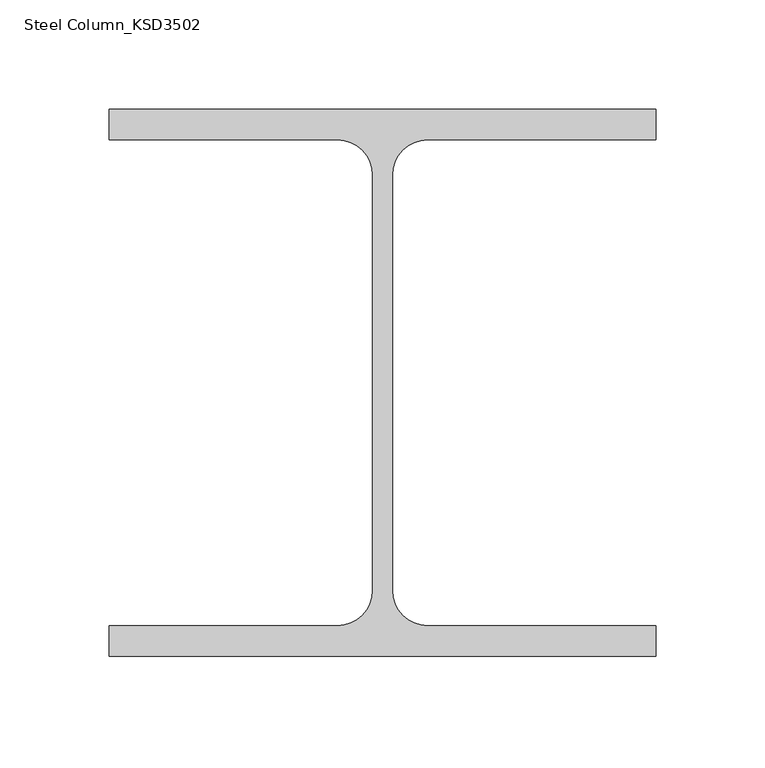
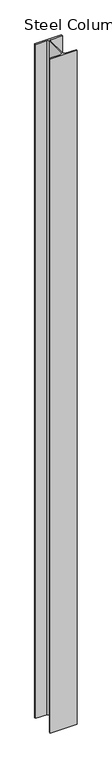
"""IFC4 building model written with IfcOpenShell, lengths in millimetres: column geometry, Steel Column_KSD3502 : H_SC_ASC_H-250×250x9x14."""

import ifcopenshell
import ifcopenshell.guid

model = None  # the IFC model being written
_history = None  # IfcOwnerHistory: only IFC2X3 demands one
_inside = {}  # id of a spatial element -> (the spatial element, [elements in it])
_under = {}  # id of a project, library or spatial element -> (it, [spatial elements below it])
_declared = {}  # id of a project -> (the project, [libraries it declares])
_typed = {}  # id of a type object -> (the type object, [elements of that type])
_made_of = {}  # id of a material, layer set ... -> (it, [elements and type objects made of it])


def new_model(schema):
    """Start an empty IFC model of exactly this schema.

    Asked for "IFC4X3", IfcOpenShell would pick the latest addendum, in which some entities
    have other attributes; the version numbers below select the first issue.
    IFC2X3 requires an IfcOwnerHistory on every rooted entity: one is made here for all.
    """
    global model, _history
    if schema == "IFC4X3":
        model = ifcopenshell.file(schema_version=(4, 3, 0, 0))
    else:
        model = ifcopenshell.file(schema=schema)
    _inside.clear()
    _under.clear()
    _declared.clear()
    _typed.clear()
    _made_of.clear()
    _history = None
    if model.schema == "IFC2X3":
        org = make("IfcOrganization", Name="unknown")
        user = make(
            "IfcPersonAndOrganization",
            ThePerson=make("IfcPerson", FamilyName="unknown"),
            TheOrganization=org,
        )
        app = make(
            "IfcApplication",
            ApplicationDeveloper=org,
            Version="unknown",
            ApplicationFullName="unknown",
            ApplicationIdentifier="unknown",
        )
        _history = make(
            "IfcOwnerHistory",
            OwningUser=user,
            OwningApplication=app,
            ChangeAction="ADDED",
            CreationDate=0,
        )
    return model


def make(cls, **values):
    """One entity of the class cls with the attributes given. An attribute that is None is left unset."""
    return model.create_entity(
        cls, **{name: value for name, value in values.items() if value is not None}
    )


def rooted(cls, **values):
    """An entity with a GlobalId (a new one), such as an element, a storey or a relation."""
    return make(cls, GlobalId=ifcopenshell.guid.new(), OwnerHistory=_history, **values)


def si_unit(unit_type, name, prefix=None):
    """IfcSIUnit, for example si_unit("LENGTHUNIT", "METRE", prefix="MILLI")."""
    return make("IfcSIUnit", UnitType=unit_type, Prefix=prefix, Name=name)


def assignment(units):
    """IfcUnitAssignment: the units of a project."""
    return None if units is None else make("IfcUnitAssignment", Units=units)


def point(xyz):
    """IfcCartesianPoint."""
    return None if xyz is None else make("IfcCartesianPoint", Coordinates=xyz)


def direction(xyz):
    """IfcDirection."""
    return None if xyz is None else make("IfcDirection", DirectionRatios=xyz)


def frame(location, z_axis=None, x_axis=None):
    """IfcAxis2Placement3D, a coordinate frame: its origin and axes. An axis left out is left unset."""
    return make(
        "IfcAxis2Placement3D",
        Location=point(location),
        Axis=direction(z_axis),
        RefDirection=direction(x_axis),
    )


def frame_2d(location, x_axis=None):
    """IfcAxis2Placement2D, a coordinate frame in the plane: its origin and x axis."""
    return make(
        "IfcAxis2Placement2D", Location=point(location), RefDirection=direction(x_axis)
    )


def origin():
    """The frame at (0, 0, 0) with its axes left unset."""
    return frame((0.0, 0.0, 0.0))


def place(relative_to, where):
    """IfcLocalPlacement: puts the frame where relative to a parent placement (None: the world)."""
    return make(
        "IfcLocalPlacement", PlacementRelTo=relative_to, RelativePlacement=where
    )


def context(
    kind, dimensions, precision=None, world=None, true_north=None, identifier=None
):
    """IfcGeometricRepresentationContext, for example the 3D "Model" context."""
    return make(
        "IfcGeometricRepresentationContext",
        ContextIdentifier=identifier,
        ContextType=kind,
        CoordinateSpaceDimension=dimensions,
        Precision=precision,
        WorldCoordinateSystem=world,
        TrueNorth=true_north,
    )


def project(units=None, contexts=None):
    """IfcProject with its units and contexts."""
    return rooted(
        "IfcProject",
        Name="project",
        RepresentationContexts=contexts,
        UnitsInContext=assignment(units),
    )


def spatial(cls, under=None, at=None, **own):
    """A site, building, storey or space (cls), placed at a placement, below another one or the project."""
    s = rooted(cls, ObjectPlacement=at, **own)
    if under is not None:
        _under.setdefault(under.id(), (under, []))[1].append(s)
    return s


def polyline(points):
    """IfcPolyline through the points."""
    return make("IfcPolyline", Points=[point(p) for p in points])


def circle_curve(where, radius):
    """IfcCircle in the frame where."""
    return make("IfcCircle", Position=where, Radius=radius)


def trimmed(basis, trim1, trim2, sense, master):
    """IfcTrimmedCurve: the piece of a basis curve between two trims."""
    return make(
        "IfcTrimmedCurve",
        BasisCurve=basis,
        Trim1=trim1,
        Trim2=trim2,
        SenseAgreement=sense,
        MasterRepresentation=master,
    )


def segment(curve, same_sense, transition):
    """IfcCompositeCurveSegment."""
    return make(
        "IfcCompositeCurveSegment",
        Transition=transition,
        SameSense=same_sense,
        ParentCurve=curve,
    )


def composite_curve(segments, self_intersect=None):
    """IfcCompositeCurve: segments joined end to end."""
    return make("IfcCompositeCurve", Segments=segments, SelfIntersect=self_intersect)


def outline(outer, holes=None, kind="AREA"):
    """IfcArbitraryClosedProfileDef: a profile drawn as a closed curve; with holes, ...WithVoids."""
    if holes is None:
        return make("IfcArbitraryClosedProfileDef", ProfileType=kind, OuterCurve=outer)
    return make(
        "IfcArbitraryProfileDefWithVoids",
        ProfileType=kind,
        OuterCurve=outer,
        InnerCurves=holes,
    )


def extrude(swept, where, along, depth):
    """IfcExtrudedAreaSolid: the profile swept, set in the frame where, extruded along a direction by depth."""
    return make(
        "IfcExtrudedAreaSolid",
        SweptArea=swept,
        Position=where,
        ExtrudedDirection=direction(along),
        Depth=depth,
    )


def shape(context_of_items, identifier, shape_type, items):
    """IfcShapeRepresentation: the items that make up one representation, for example the "Body"."""
    return make(
        "IfcShapeRepresentation",
        ContextOfItems=context_of_items,
        RepresentationIdentifier=identifier,
        RepresentationType=shape_type,
        Items=items,
    )


def source(mapping_origin, context_of_items, identifier, shape_type, items):
    """IfcRepresentationMap: a shape defined once, which mapped items show again and again."""
    return make(
        "IfcRepresentationMap",
        MappingOrigin=mapping_origin,
        MappedRepresentation=shape(context_of_items, identifier, shape_type, items),
    )


def transform(
    local_origin,
    x_axis=None,
    y_axis=None,
    z_axis=None,
    scale=None,
    scale2=None,
    scale3=None,
    uniform=True,
):
    """IfcCartesianTransformationOperator3D, or its non-uniform kind. x_axis, y_axis, z_axis: its Axis1, 2, 3."""
    if uniform:
        return make(
            "IfcCartesianTransformationOperator3D",
            Axis1=direction(x_axis),
            Axis2=direction(y_axis),
            LocalOrigin=point(local_origin),
            Scale=scale,
            Axis3=direction(z_axis),
        )
    return make(
        "IfcCartesianTransformationOperator3DnonUniform",
        Axis1=direction(x_axis),
        Axis2=direction(y_axis),
        LocalOrigin=point(local_origin),
        Scale=scale,
        Axis3=direction(z_axis),
        Scale2=scale2,
        Scale3=scale3,
    )


def mapped(mapping_source, mapping_target):
    """IfcMappedItem: shows the shape of a source again, moved by a transform."""
    return make(
        "IfcMappedItem", MappingSource=mapping_source, MappingTarget=mapping_target
    )


def made_of(thing, what):
    """Note that an element or type object is made of a material, layer set ...; save() writes the relation."""
    if what is not None:
        _made_of.setdefault(what.id(), (what, []))[1].append(thing)
    return thing


def element(
    cls,
    number,
    at=None,
    inside=None,
    cuts=None,
    type_object=None,
    material=None,
    context=None,
    identifier="Body",
    shape_type=None,
    held_by="IfcProductDefinitionShape",
    body=None,
    shapes=None,
    **own,
):
    """One element of the class cls, such as IfcWall. Its Tag is "e" and its number.

    at: its placement. inside: the storey or other place that contains it. cuts: it is an
    opening in that element (IfcRelVoidsElement). A single representation is given by context,
    identifier, shape_type and body (its items); several are given by shapes. held_by: the class
    of the entity that holds the representations. save() writes the other relations.
    """
    e = rooted(cls, Tag="e%d" % number, ObjectPlacement=at, **own)
    if body is not None:
        shapes = [shape(context, identifier, shape_type, body)]
    if shapes is not None:
        e.Representation = make(held_by, Representations=shapes)
    if inside is not None:
        _inside.setdefault(inside.id(), (inside, []))[1].append(e)
    if cuts is not None:
        rooted(
            "IfcRelVoidsElement", RelatingBuildingElement=cuts, RelatedOpeningElement=e
        )
    if type_object is not None:
        _typed.setdefault(type_object.id(), (type_object, []))[1].append(e)
    return made_of(e, material)


def aggregate(whole, parts):
    """IfcRelAggregates: a whole, such as a stair, and the parts it consists of."""
    return rooted("IfcRelAggregates", RelatingObject=whole, RelatedObjects=parts)


def save(model, path):
    """Write the relations noted so far, then the file.

    IfcRelAggregates (storeys below a building ...), IfcRelContainedInSpatialStructure (elements
    in a storey), IfcRelDefinesByType, IfcRelAssociatesMaterial and IfcRelDeclares: one each for
    every whole, place, type object, material and project.
    """
    for whole, parts in _under.values():
        aggregate(whole, parts)
    for where, things in _inside.values():
        rooted(
            "IfcRelContainedInSpatialStructure",
            RelatedElements=things,
            RelatingStructure=where,
        )
    for kind, things in _typed.values():
        rooted("IfcRelDefinesByType", RelatedObjects=things, RelatingType=kind)
    for what, things in _made_of.values():
        rooted("IfcRelAssociatesMaterial", RelatedObjects=things, RelatingMaterial=what)
    for by, libraries in _declared.values():
        rooted("IfcRelDeclares", RelatingContext=by, RelatedDefinitions=libraries)
    model.write(path)


def steel_column_ksd3502_8fa00422(model_context):
    return source(origin(), model_context, "Body", "SweptSolid", [
        extrude(outline(composite_curve([segment(polyline([(125.0, 125.0), (125.0, 111.0), (20.5, 111.0)]), True, "CONTINUOUS"), segment(trimmed(circle_curve(frame_2d((20.5, 95.0)), 16.0), [point((20.5, 111.0))], [point((4.5, 95.0))], True, "CARTESIAN"), True, "CONTINUOUS"), segment(polyline([(4.5, 95.0), (4.5, -95.0)]), True, "CONTINUOUS"), segment(trimmed(circle_curve(frame_2d((20.5, -95.0)), 16.0), [point((4.5, -95.0))], [point((20.5, -111.0))], True, "CARTESIAN"), True, "CONTINUOUS"), segment(polyline([(20.5, -111.0), (125.0, -111.0), (125.0, -125.0), (-125.0, -125.0), (-125.0, -111.0), (-20.5, -111.0)]), True, "CONTINUOUS"), segment(trimmed(circle_curve(frame_2d((-20.5, -95.0)), 16.0), [point((-20.5, -111.0))], [point((-4.5, -95.0))], True, "CARTESIAN"), True, "CONTINUOUS"), segment(polyline([(-4.5, -95.0), (-4.5, 95.0)]), True, "CONTINUOUS"), segment(trimmed(circle_curve(frame_2d((-20.5, 95.0)), 16.0), [point((-4.5, 95.0))], [point((-20.5, 111.0))], True, "CARTESIAN"), True, "CONTINUOUS"), segment(polyline([(-20.5, 111.0), (-125.0, 111.0), (-125.0, 125.0), (125.0, 125.0)]), True, "CONTINUOUS")], self_intersect=False)), frame((0.0, 0.0, 599.9720055), z_axis=(0.0, 0.0, 1.0), x_axis=(1.0, 0.0, 0.0)), (0.0, 0.0, 1.0), 6600.0),
    ])


if __name__ == "__main__":
    model = new_model("IFC4")
    model_context = context("Model", 3, world=origin())
    ifc_project = project(units=[si_unit("LENGTHUNIT", "METRE", prefix="MILLI")], contexts=[model_context])
    site = spatial("IfcSite", under=ifc_project)
    building = spatial("IfcBuilding", under=site)
    placement = place(None, origin())
    steel_column_ksd3502_shape = steel_column_ksd3502_8fa00422(model_context)
    element("IfcColumn", 1, ObjectType="Steel Column_KSD3502 : H_SC_ASC_H-250×250x9x14", at=placement, inside=building, context=model_context, shape_type="MappedRepresentation", body=[
        mapped(steel_column_ksd3502_shape, transform((0.0, 0.0, 0.0), x_axis=(1.0, 0.0, 0.0), y_axis=(0.0, 1.0, 0.0), z_axis=(0.0, 0.0, 1.0))),
    ])
    save(model, "model.ifc")

# Revit data of these elements
# Type "Steel Column_KSD3502 : H_SC_ASC_H-250×250x9x14"
#   Width = 25.0 cm
#   Web Thickness = 0.9 cm
#   Web Fillet = 1.6 cm
#   Warping Constant = 507646.0 cm⁶
#   Torsional Moment of Inertia = 51.4681 cm⁴
#   Section Area = 92.18 cm²
#   Plastic Modulus weak axis = 444.0 cm³
#   Plastic Modulus strong axis = 960.0 cm³
#   Perimeter = 1.27 m²/m
#   Nominal Weight = 72.40 kgf/m
#   Moment of Inertia weak axis = 3650.00 cm⁴
#   Moment of Inertia strong axis = 10800.00 cm⁴
#   Height = 25.0 cm
#   Flange Thickness = 1.4 cm
#   Elastic Modulus weak axis = 292.0 cm³
#   Elastic Modulus strong axis = 867.0 cm³
#   Centroid Vertical = 12.5 cm
#   Centroid Horizontal = 12.5 cm
#   Bolt Spacing = 13.97 cm
#   Structural Material [instance default] = Steel, 45-345
#   Section Name Key = ""
#   Assembly Code = ""
# Element 1 (IfcColumn, "Steel Column_KSD3502 : H_SC_ASC_H-250×250x9x14")
#   Structural Material = A03AD029-00005_Anchor Bolt (Installation only)_M24
#   Materials on its faces: "A03AD029-00005_Anchor Bolt (Installation only)_M24"
# Materials
#   "Steel, 45-345": class "Metal", colour RGB 189 187 185, transparency 0, Description = "Steel 345 MPa", Cost = 0
#   "A03AD029-00005_Anchor Bolt (Installation only)_M24": class "Unassigned", colour RGB 84 83 81, transparency 0, Cost = 0
